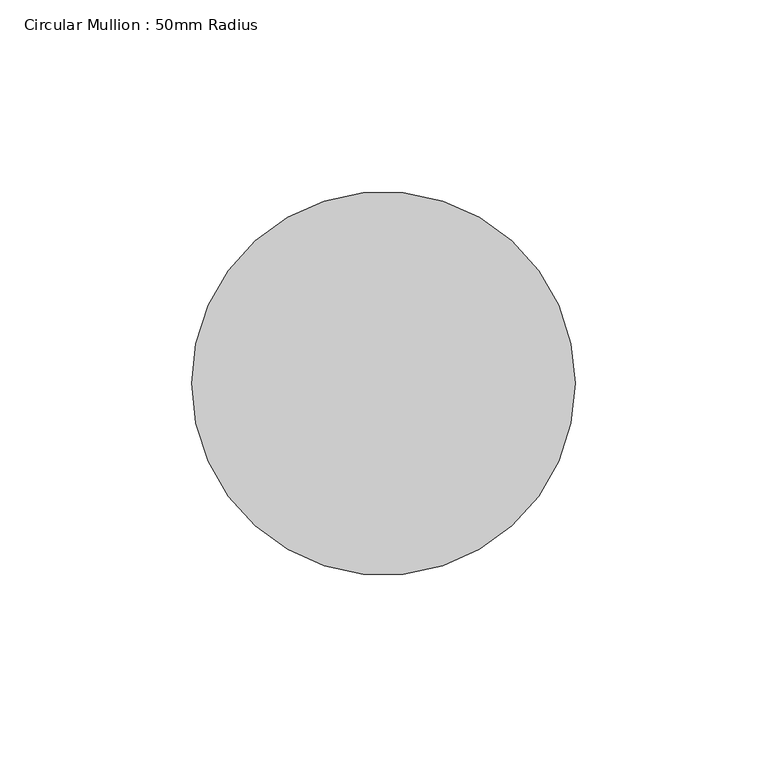
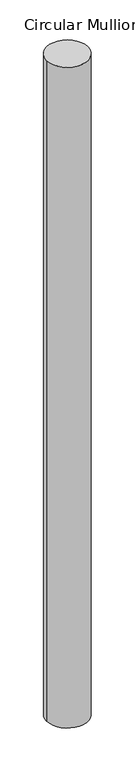
"""IFC4 building model written with IfcOpenShell, lengths in millimetres: member geometry, Circular Mullion : 50mm Radius."""

from ifc_helpers import new_model, si_unit, point, frame, origin, origin_2d, place, context, project, spatial, circle_curve, trimmed, segment, composite_curve, outline, extrude, source, transform, mapped, element, save


def circular_mullion_50mm_radius_6a153160(model_context):
    return source(origin(), model_context, "Body", "SweptSolid", [
        extrude(outline(composite_curve([segment(trimmed(circle_curve(origin_2d(), 50.0), [point((50.0, 0.0))], [point((-50.0, 0.0))], False, "CARTESIAN"), True, "CONTINUOUS"), segment(trimmed(circle_curve(origin_2d(), 50.0), [point((-50.0, 0.0))], [point((50.0, 0.0))], False, "CARTESIAN"), True, "CONTINUOUS")], self_intersect=False)), frame((0.0, 0.0, -1685.660868), z_axis=(0.0, 0.0, 1.0), x_axis=(1.0, 0.0, 0.0)), (0.0, 0.0, 1.0), 1685.660868),
    ])


if __name__ == "__main__":
    model = new_model("IFC4")
    model_context = context("Model", 3, world=origin())
    ifc_project = project(units=[si_unit("LENGTHUNIT", "METRE", prefix="MILLI")], contexts=[model_context])
    site = spatial("IfcSite", under=ifc_project)
    building = spatial("IfcBuilding", under=site)
    placement = place(None, origin())
    circular_mullion_50mm_radius_shape = circular_mullion_50mm_radius_6a153160(model_context)
    element("IfcMember", 1, ObjectType="Circular Mullion : 50mm Radius", at=placement, inside=building, context=model_context, shape_type="MappedRepresentation", body=[
        mapped(circular_mullion_50mm_radius_shape, transform((0.0, 0.0, 0.0), x_axis=(1.0, 0.0, 0.0), y_axis=(0.0, 1.0, 0.0), z_axis=(0.0, 0.0, 1.0))),
    ])
    save(model, "model.ifc")

# Revit data of these elements
# Type "Circular Mullion : 50mm Radius"
#   built-in parameter 1007350 = 0.164042 (stored number, unit not read)
# Element 1 (IfcMember, "Circular Mullion : 50mm Radius")
#   Materials on its faces: "Aluminium"
# Materials
#   "Aluminium": class "Metal", colour RGB 247 247 247, transparency 0, Description = "Aluminium 6061", Cost = 0
